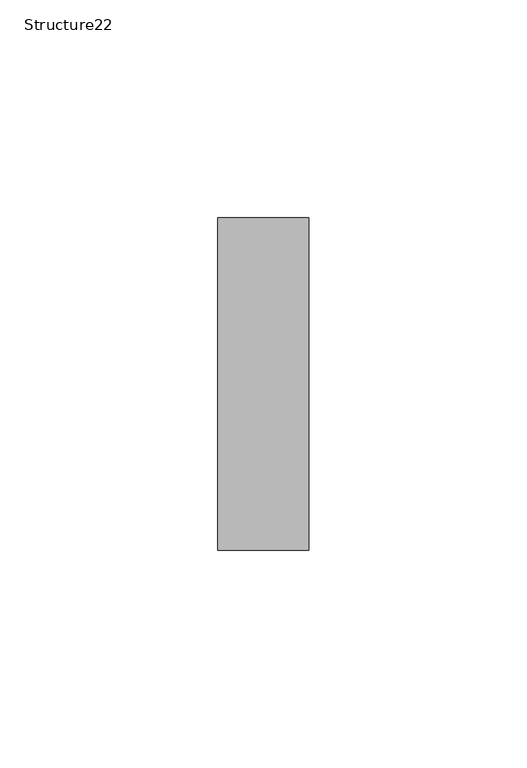
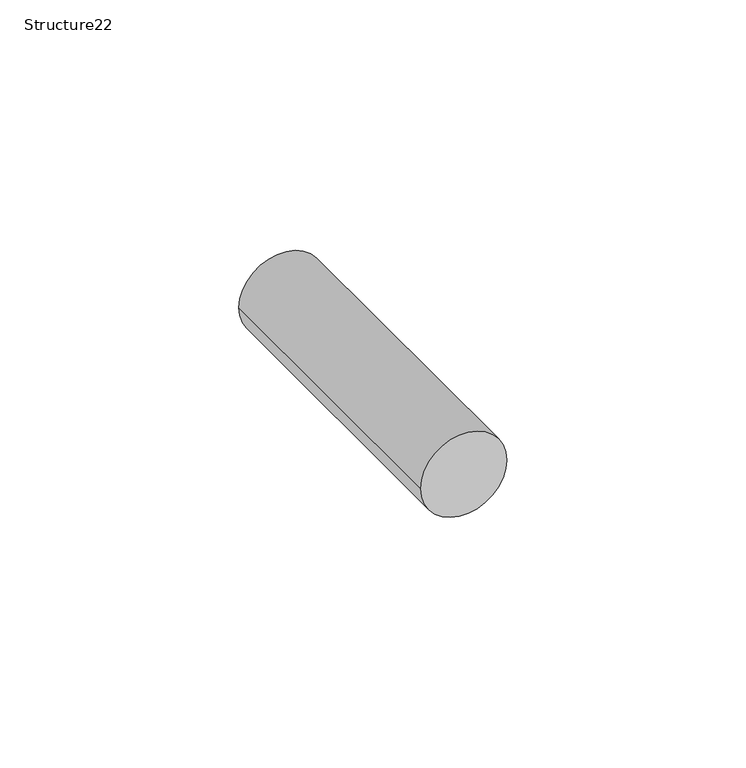
"""IFC4 building model written with IfcOpenShell, lengths in millimetres: proxy geometry, Structure22 : Structure668217150."""

from ifc_helpers import new_model, si_unit, point, frame, frame_2d, origin, place, context, project, spatial, circle_curve, trimmed, segment, composite_curve, outline, extrude, source, transform, mapped, element, save


def structure22_d75082ea(model_context):
    return source(origin(), model_context, "Body", "SweptSolid", [
        extrude(outline(composite_curve([segment(trimmed(circle_curve(frame_2d((40908.7088339, 9847.8795269)), 10.4009751), [point((40908.7088339, 9837.4785517))], [point((40908.7088339, 9858.280502))], False, "CARTESIAN"), True, "CONTINUOUS"), segment(trimmed(circle_curve(frame_2d((40908.7088339, 9847.8795269)), 10.4009751), [point((40908.7088339, 9858.280502))], [point((40908.7088339, 9837.4785517))], False, "CARTESIAN"), True, "CONTINUOUS")], self_intersect=False)), frame((0.0, 1837.2573723, 0.0), z_axis=(0.0, 1.0, 0.0), x_axis=(0.0, 0.0, 1.0)), (0.0, 0.0, 1.0), 76.2),
    ])


if __name__ == "__main__":
    model = new_model("IFC4")
    model_context = context("Model", 3, world=origin())
    ifc_project = project(units=[si_unit("LENGTHUNIT", "METRE", prefix="MILLI")], contexts=[model_context])
    site = spatial("IfcSite", under=ifc_project)
    building = spatial("IfcBuilding", under=site)
    placement = place(None, origin())
    structure22_shape = structure22_d75082ea(model_context)
    element("IfcBuildingElementProxy", 1, Name="Structure22 : Structure668217150", ObjectType="Structure22 : Structure668217150", at=placement, inside=building, context=model_context, shape_type="MappedRepresentation", body=[
        mapped(structure22_shape, transform((0.0, 0.0, 0.0), x_axis=(1.0, 0.0, 0.0), y_axis=(0.0, 1.0, 0.0), z_axis=(0.0, 0.0, 1.0))),
    ])
    save(model, "model.ifc")

# Revit data of these elements
# Type "Structure22 : Structure668217150"
#   NameOverride = "Structure668217150"
# Element 1 (IfcBuildingElementProxy, "Structure22 : Structure668217150")
#   Materials on its faces: "1.5\" DIA. STAINLESS STEEL RAILING"
# Materials
#   "1.5\" DIA. STAINLESS STEEL RAILING": class "Unassigned", colour RGB 128 128 128, transparency 0, Cost = 0
